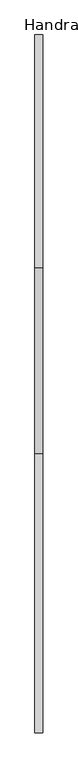
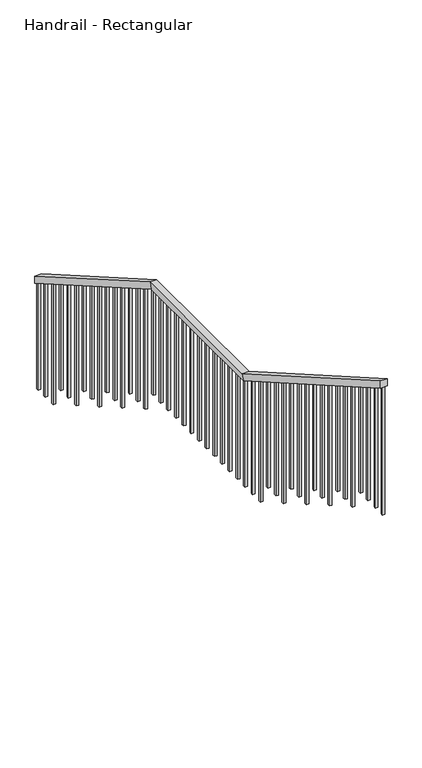
"""IFC4 building model written with IfcOpenShell, lengths in millimetres: railing geometry, Handrail - Rectangular."""

from ifc_helpers import new_model, si_unit, frame, origin, place, context, project, spatial, polyline, outline, extrude, faceted_brep, source, transform, mapped, element, save


def handrail_rectangular_dd9c5432(model_context):
    return source(origin(), model_context, "Body", "SolidModel", [
        faceted_brep([(-91816.1359, 4699.0, 12280.8850588), (-91765.3359, 4699.0, 12280.8850588), (-91765.3359, 4699.0, 12222.2920825), (-91816.1359, 4699.0, 12222.2920825), (-91816.1359, 3175.0, 13156.8115294), (-91765.3359, 3175.0, 13156.8115294), (-91765.3359, 3161.4412183, 13106.0115294), (-91816.1359, 3161.4412183, 13106.0115294), (-91816.1359, 1955.8, 13156.8115294), (-91765.3359, 1955.8, 13156.8115294), (-91765.3359, 1942.2412183, 13106.0115294), (-91816.1359, 1942.2412183, 13106.0115294), (-91816.1359, 127.0, 14207.9232941), (-91816.1359, 127.0, 14149.3303178), (-91765.3359, 127.0, 14149.3303178), (-91765.3359, 127.0, 14207.9232941)], [[[0, 1, 2, 3]], [[1, 0, 4, 5]], [[2, 1, 5, 6]], [[3, 2, 6, 7]], [[0, 3, 7, 4]], [[5, 4, 8, 9]], [[6, 5, 9, 10]], [[7, 6, 10, 11]], [[4, 7, 11, 8]], [[12, 13, 14, 15]], [[9, 8, 12, 15]], [[10, 9, 15, 14]], [[11, 10, 14, 13]], [[8, 11, 13, 12]]]),
        extrude(outline(polyline([(219.075, 14096.4097602), (238.125, 14085.4606794), (238.125, 13118.338), (219.075, 13118.338), (219.075, 14096.4097602)])), frame((-91800.2609, 0.0, 0.0), z_axis=(1.0, 0.0, 0.0), x_axis=(0.0, 1.0, 0.0)), (0.0, 0.0, 1.0), 19.05),
        extrude(outline(polyline([(320.675, 14038.0146622), (339.725, 14027.0655813), (339.725, 13118.338), (320.675, 13118.338), (320.675, 14038.0146622)])), frame((-91800.2609, 0.0, 0.0), z_axis=(1.0, 0.0, 0.0), x_axis=(0.0, 1.0, 0.0)), (0.0, 0.0, 1.0), 19.05),
        extrude(outline(polyline([(422.275, 13979.6195642), (441.325, 13968.6704833), (441.325, 13118.338), (422.275, 13118.338), (422.275, 13979.6195642)])), frame((-91800.2609, 0.0, 0.0), z_axis=(1.0, 0.0, 0.0), x_axis=(0.0, 1.0, 0.0)), (0.0, 0.0, 1.0), 19.05),
        extrude(outline(polyline([(523.875, 13921.2244661), (542.925, 13910.2753852), (542.925, 12943.1527059), (523.875, 12943.1527059), (523.875, 13921.2244661)])), frame((-91800.2609, 0.0, 0.0), z_axis=(1.0, 0.0, 0.0), x_axis=(0.0, 1.0, 0.0)), (0.0, 0.0, 1.0), 19.05),
        extrude(outline(polyline([(625.475, 13862.8293681), (644.525, 13851.8802872), (644.525, 12943.1527059), (625.475, 12943.1527059), (625.475, 13862.8293681)])), frame((-91800.2609, 0.0, 0.0), z_axis=(1.0, 0.0, 0.0), x_axis=(0.0, 1.0, 0.0)), (0.0, 0.0, 1.0), 19.05),
        extrude(outline(polyline([(727.075, 13804.43427), (746.125, 13793.4851892), (746.125, 12943.1527059), (727.075, 12943.1527059), (727.075, 13804.43427)])), frame((-91800.2609, 0.0, 0.0), z_axis=(1.0, 0.0, 0.0), x_axis=(0.0, 1.0, 0.0)), (0.0, 0.0, 1.0), 19.05),
        extrude(outline(polyline([(828.675, 13746.039172), (847.725, 13735.0900911), (847.725, 12767.9674118), (828.675, 12767.9674118), (828.675, 13746.039172)])), frame((-91800.2609, 0.0, 0.0), z_axis=(1.0, 0.0, 0.0), x_axis=(0.0, 1.0, 0.0)), (0.0, 0.0, 1.0), 19.05),
        extrude(outline(polyline([(930.275, 13687.644074), (949.325, 13676.6949931), (949.325, 12767.9674118), (930.275, 12767.9674118), (930.275, 13687.644074)])), frame((-91800.2609, 0.0, 0.0), z_axis=(1.0, 0.0, 0.0), x_axis=(0.0, 1.0, 0.0)), (0.0, 0.0, 1.0), 19.05),
        extrude(outline(polyline([(1031.875, 13629.2489759), (1050.925, 13618.299895), (1050.925, 12767.9674118), (1031.875, 12767.9674118), (1031.875, 13629.2489759)])), frame((-91800.2609, 0.0, 0.0), z_axis=(1.0, 0.0, 0.0), x_axis=(0.0, 1.0, 0.0)), (0.0, 0.0, 1.0), 19.05),
        extrude(outline(polyline([(1133.475, 13570.8538779), (1152.525, 13559.904797), (1152.525, 12592.7821176), (1133.475, 12592.7821176), (1133.475, 13570.8538779)])), frame((-91800.2609, 0.0, 0.0), z_axis=(1.0, 0.0, 0.0), x_axis=(0.0, 1.0, 0.0)), (0.0, 0.0, 1.0), 19.05),
        extrude(outline(polyline([(1235.075, 13512.4587799), (1254.125, 13501.509699), (1254.125, 12592.7821176), (1235.075, 12592.7821176), (1235.075, 13512.4587799)])), frame((-91800.2609, 0.0, 0.0), z_axis=(1.0, 0.0, 0.0), x_axis=(0.0, 1.0, 0.0)), (0.0, 0.0, 1.0), 19.05),
        extrude(outline(polyline([(1336.675, 13454.0636818), (1355.725, 13443.1146009), (1355.725, 12592.7821176), (1336.675, 12592.7821176), (1336.675, 13454.0636818)])), frame((-91800.2609, 0.0, 0.0), z_axis=(1.0, 0.0, 0.0), x_axis=(0.0, 1.0, 0.0)), (0.0, 0.0, 1.0), 19.05),
        extrude(outline(polyline([(1438.275, 13395.6685838), (1457.325, 13384.7195029), (1457.325, 12417.5968235), (1438.275, 12417.5968235), (1438.275, 13395.6685838)])), frame((-91800.2609, 0.0, 0.0), z_axis=(1.0, 0.0, 0.0), x_axis=(0.0, 1.0, 0.0)), (0.0, 0.0, 1.0), 19.05),
        extrude(outline(polyline([(1539.875, 13337.2734857), (1558.925, 13326.3244049), (1558.925, 12417.5968235), (1539.875, 12417.5968235), (1539.875, 13337.2734857)])), frame((-91800.2609, 0.0, 0.0), z_axis=(1.0, 0.0, 0.0), x_axis=(0.0, 1.0, 0.0)), (0.0, 0.0, 1.0), 19.05),
        extrude(outline(polyline([(1641.475, 13278.8783877), (1660.525, 13267.9293068), (1660.525, 12417.5968235), (1641.475, 12417.5968235), (1641.475, 13278.8783877)])), frame((-91800.2609, 0.0, 0.0), z_axis=(1.0, 0.0, 0.0), x_axis=(0.0, 1.0, 0.0)), (0.0, 0.0, 1.0), 19.05),
        extrude(outline(polyline([(1743.075, 13220.4832897), (1762.125, 13209.5342088), (1762.125, 12242.4115294), (1743.075, 12242.4115294), (1743.075, 13220.4832897)])), frame((-91800.2609, 0.0, 0.0), z_axis=(1.0, 0.0, 0.0), x_axis=(0.0, 1.0, 0.0)), (0.0, 0.0, 1.0), 19.05),
        extrude(outline(polyline([(1844.675, 13162.0881916), (1863.725, 13151.1391107), (1863.725, 12242.4115294), (1844.675, 12242.4115294), (1844.675, 13162.0881916)])), frame((-91800.2609, 0.0, 0.0), z_axis=(1.0, 0.0, 0.0), x_axis=(0.0, 1.0, 0.0)), (0.0, 0.0, 1.0), 19.05),
        extrude(outline(polyline([(-91800.2609, 2066.925), (-91781.2109, 2066.925), (-91781.2109, 2047.875), (-91800.2609, 2047.875), (-91800.2609, 2066.925)])), frame((0.0, 0.0, 12242.4115294), z_axis=(0.0, 0.0, 1.0), x_axis=(1.0, 0.0, 0.0)), (0.0, 0.0, 1.0), 863.6),
        extrude(outline(polyline([(-91800.2609, 2168.525), (-91781.2109, 2168.525), (-91781.2109, 2149.475), (-91800.2609, 2149.475), (-91800.2609, 2168.525)])), frame((0.0, 0.0, 12242.4115294), z_axis=(0.0, 0.0, 1.0), x_axis=(1.0, 0.0, 0.0)), (0.0, 0.0, 1.0), 863.6),
        extrude(outline(polyline([(-91800.2609, 2270.125), (-91781.2109, 2270.125), (-91781.2109, 2251.075), (-91800.2609, 2251.075), (-91800.2609, 2270.125)])), frame((0.0, 0.0, 12242.4115294), z_axis=(0.0, 0.0, 1.0), x_axis=(1.0, 0.0, 0.0)), (0.0, 0.0, 1.0), 863.6),
        extrude(outline(polyline([(-91800.2609, 2371.725), (-91781.2109, 2371.725), (-91781.2109, 2352.675), (-91800.2609, 2352.675), (-91800.2609, 2371.725)])), frame((0.0, 0.0, 12242.4115294), z_axis=(0.0, 0.0, 1.0), x_axis=(1.0, 0.0, 0.0)), (0.0, 0.0, 1.0), 863.6),
        extrude(outline(polyline([(-91800.2609, 2473.325), (-91781.2109, 2473.325), (-91781.2109, 2454.275), (-91800.2609, 2454.275), (-91800.2609, 2473.325)])), frame((0.0, 0.0, 12242.4115294), z_axis=(0.0, 0.0, 1.0), x_axis=(1.0, 0.0, 0.0)), (0.0, 0.0, 1.0), 863.6),
        extrude(outline(polyline([(-91800.2609, 2574.925), (-91781.2109, 2574.925), (-91781.2109, 2555.875), (-91800.2609, 2555.875), (-91800.2609, 2574.925)])), frame((0.0, 0.0, 12242.4115294), z_axis=(0.0, 0.0, 1.0), x_axis=(1.0, 0.0, 0.0)), (0.0, 0.0, 1.0), 863.6),
        extrude(outline(polyline([(-91800.2609, 2676.525), (-91781.2109, 2676.525), (-91781.2109, 2657.475), (-91800.2609, 2657.475), (-91800.2609, 2676.525)])), frame((0.0, 0.0, 12242.4115294), z_axis=(0.0, 0.0, 1.0), x_axis=(1.0, 0.0, 0.0)), (0.0, 0.0, 1.0), 863.6),
        extrude(outline(polyline([(-91800.2609, 2778.125), (-91781.2109, 2778.125), (-91781.2109, 2759.075), (-91800.2609, 2759.075), (-91800.2609, 2778.125)])), frame((0.0, 0.0, 12242.4115294), z_axis=(0.0, 0.0, 1.0), x_axis=(1.0, 0.0, 0.0)), (0.0, 0.0, 1.0), 863.6),
        extrude(outline(polyline([(-91800.2609, 2879.725), (-91781.2109, 2879.725), (-91781.2109, 2860.675), (-91800.2609, 2860.675), (-91800.2609, 2879.725)])), frame((0.0, 0.0, 12242.4115294), z_axis=(0.0, 0.0, 1.0), x_axis=(1.0, 0.0, 0.0)), (0.0, 0.0, 1.0), 863.6),
        extrude(outline(polyline([(-91800.2609, 2981.325), (-91781.2109, 2981.325), (-91781.2109, 2962.275), (-91800.2609, 2962.275), (-91800.2609, 2981.325)])), frame((0.0, 0.0, 12242.4115294), z_axis=(0.0, 0.0, 1.0), x_axis=(1.0, 0.0, 0.0)), (0.0, 0.0, 1.0), 863.6),
        extrude(outline(polyline([(-91800.2609, 3082.925), (-91781.2109, 3082.925), (-91781.2109, 3063.875), (-91800.2609, 3063.875), (-91800.2609, 3082.925)])), frame((0.0, 0.0, 12242.4115294), z_axis=(0.0, 0.0, 1.0), x_axis=(1.0, 0.0, 0.0)), (0.0, 0.0, 1.0), 863.6),
        extrude(outline(polyline([(3267.075, 13045.2979955), (3286.125, 13034.3489147), (3286.125, 12067.2262353), (3267.075, 12067.2262353), (3267.075, 13045.2979955)])), frame((-91800.2609, 0.0, 0.0), z_axis=(1.0, 0.0, 0.0), x_axis=(0.0, 1.0, 0.0)), (0.0, 0.0, 1.0), 19.05),
        extrude(outline(polyline([(3368.675, 12986.9028975), (3387.725, 12975.9538166), (3387.725, 12067.2262353), (3368.675, 12067.2262353), (3368.675, 12986.9028975)])), frame((-91800.2609, 0.0, 0.0), z_axis=(1.0, 0.0, 0.0), x_axis=(0.0, 1.0, 0.0)), (0.0, 0.0, 1.0), 19.05),
        extrude(outline(polyline([(3470.275, 12928.5077995), (3489.325, 12917.5587186), (3489.325, 12067.2262353), (3470.275, 12067.2262353), (3470.275, 12928.5077995)])), frame((-91800.2609, 0.0, 0.0), z_axis=(1.0, 0.0, 0.0), x_axis=(0.0, 1.0, 0.0)), (0.0, 0.0, 1.0), 19.05),
        extrude(outline(polyline([(3571.875, 12870.1127014), (3590.925, 12859.1636205), (3590.925, 11892.0409412), (3571.875, 11892.0409412), (3571.875, 12870.1127014)])), frame((-91800.2609, 0.0, 0.0), z_axis=(1.0, 0.0, 0.0), x_axis=(0.0, 1.0, 0.0)), (0.0, 0.0, 1.0), 19.05),
        extrude(outline(polyline([(3673.475, 12811.7176034), (3692.525, 12800.7685225), (3692.525, 11892.0409412), (3673.475, 11892.0409412), (3673.475, 12811.7176034)])), frame((-91800.2609, 0.0, 0.0), z_axis=(1.0, 0.0, 0.0), x_axis=(0.0, 1.0, 0.0)), (0.0, 0.0, 1.0), 19.05),
        extrude(outline(polyline([(3775.075, 12753.3225053), (3794.125, 12742.3734245), (3794.125, 11892.0409412), (3775.075, 11892.0409412), (3775.075, 12753.3225053)])), frame((-91800.2609, 0.0, 0.0), z_axis=(1.0, 0.0, 0.0), x_axis=(0.0, 1.0, 0.0)), (0.0, 0.0, 1.0), 19.05),
        extrude(outline(polyline([(3876.675, 12694.9274073), (3895.725, 12683.9783264), (3895.725, 11716.8556471), (3876.675, 11716.8556471), (3876.675, 12694.9274073)])), frame((-91800.2609, 0.0, 0.0), z_axis=(1.0, 0.0, 0.0), x_axis=(0.0, 1.0, 0.0)), (0.0, 0.0, 1.0), 19.05),
        extrude(outline(polyline([(3978.275, 12636.5323093), (3997.325, 12625.5832284), (3997.325, 11716.8556471), (3978.275, 11716.8556471), (3978.275, 12636.5323093)])), frame((-91800.2609, 0.0, 0.0), z_axis=(1.0, 0.0, 0.0), x_axis=(0.0, 1.0, 0.0)), (0.0, 0.0, 1.0), 19.05),
        extrude(outline(polyline([(4079.875, 12578.1372112), (4098.925, 12567.1881303), (4098.925, 11716.8556471), (4079.875, 11716.8556471), (4079.875, 12578.1372112)])), frame((-91800.2609, 0.0, 0.0), z_axis=(1.0, 0.0, 0.0), x_axis=(0.0, 1.0, 0.0)), (0.0, 0.0, 1.0), 19.05),
        extrude(outline(polyline([(4181.475, 12519.7421132), (4200.525, 12508.7930323), (4200.525, 11541.6703529), (4181.475, 11541.6703529), (4181.475, 12519.7421132)])), frame((-91800.2609, 0.0, 0.0), z_axis=(1.0, 0.0, 0.0), x_axis=(0.0, 1.0, 0.0)), (0.0, 0.0, 1.0), 19.05),
        extrude(outline(polyline([(4283.075, 12461.3470151), (4302.125, 12450.3979343), (4302.125, 11541.6703529), (4283.075, 11541.6703529), (4283.075, 12461.3470151)])), frame((-91800.2609, 0.0, 0.0), z_axis=(1.0, 0.0, 0.0), x_axis=(0.0, 1.0, 0.0)), (0.0, 0.0, 1.0), 19.05),
        extrude(outline(polyline([(4384.675, 12402.9519171), (4403.725, 12392.0028362), (4403.725, 11541.6703529), (4384.675, 11541.6703529), (4384.675, 12402.9519171)])), frame((-91800.2609, 0.0, 0.0), z_axis=(1.0, 0.0, 0.0), x_axis=(0.0, 1.0, 0.0)), (0.0, 0.0, 1.0), 19.05),
        extrude(outline(polyline([(4486.275, 12344.5568191), (4505.325, 12333.6077382), (4505.325, 11366.4850588), (4486.275, 11366.4850588), (4486.275, 12344.5568191)])), frame((-91800.2609, 0.0, 0.0), z_axis=(1.0, 0.0, 0.0), x_axis=(0.0, 1.0, 0.0)), (0.0, 0.0, 1.0), 19.05),
        extrude(outline(polyline([(4587.875, 12286.161721), (4606.925, 12275.2126401), (4606.925, 11366.4850588), (4587.875, 11366.4850588), (4587.875, 12286.161721)])), frame((-91800.2609, 0.0, 0.0), z_axis=(1.0, 0.0, 0.0), x_axis=(0.0, 1.0, 0.0)), (0.0, 0.0, 1.0), 19.05),
        extrude(outline(polyline([(-91800.2609, 1965.325), (-91781.2109, 1965.325), (-91781.2109, 1946.275), (-91800.2609, 1946.275), (-91800.2609, 1965.325)])), frame((0.0, 0.0, 12242.4115294), z_axis=(0.0, 0.0, 1.0), x_axis=(1.0, 0.0, 0.0)), (0.0, 0.0, 1.0), 863.6),
        extrude(outline(polyline([(3165.475, 13103.6930936), (3184.525, 13092.7440127), (3184.525, 12242.4115294), (3165.475, 12242.4115294), (3165.475, 13103.6930936)])), frame((-91800.2609, 0.0, 0.0), z_axis=(1.0, 0.0, 0.0), x_axis=(0.0, 1.0, 0.0)), (0.0, 0.0, 1.0), 19.05),
        extrude(outline(polyline([(127.0, 14149.3303178), (146.05, 14138.381237), (146.05, 13118.338), (127.0, 13118.338), (127.0, 14149.3303178)])), frame((-91800.2609, 0.0, 0.0), z_axis=(1.0, 0.0, 0.0), x_axis=(0.0, 1.0, 0.0)), (0.0, 0.0, 1.0), 19.05),
        extrude(outline(polyline([(4679.95, 12233.2411634), (4699.0, 12222.2920825), (4699.0, 11366.4850588), (4679.95, 11366.4850588), (4679.95, 12233.2411634)])), frame((-91800.2609, 0.0, 0.0), z_axis=(1.0, 0.0, 0.0), x_axis=(0.0, 1.0, 0.0)), (0.0, 0.0, 1.0), 19.05),
    ])


if __name__ == "__main__":
    model = new_model("IFC4")
    model_context = context("Model", 3, world=origin())
    ifc_project = project(units=[si_unit("LENGTHUNIT", "METRE", prefix="MILLI")], contexts=[model_context])
    site = spatial("IfcSite", under=ifc_project)
    building = spatial("IfcBuilding", under=site)
    placement = place(None, origin())
    handrail_rectangular_shape = handrail_rectangular_dd9c5432(model_context)
    element("IfcRailing", 1, ObjectType="Handrail - Rectangular", at=placement, inside=building, context=model_context, shape_type="MappedRepresentation", body=[
        mapped(handrail_rectangular_shape, transform((0.0, 0.0, 0.0), x_axis=(1.0, 0.0, 0.0), y_axis=(0.0, 1.0, 0.0), z_axis=(0.0, 0.0, 1.0))),
    ])
    save(model, "model.ifc")
